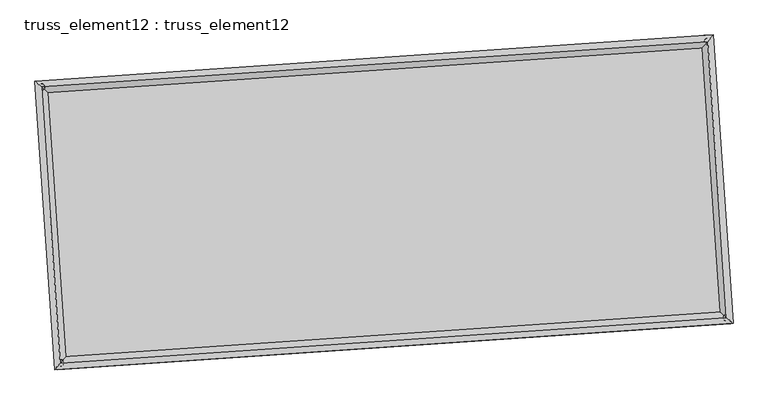
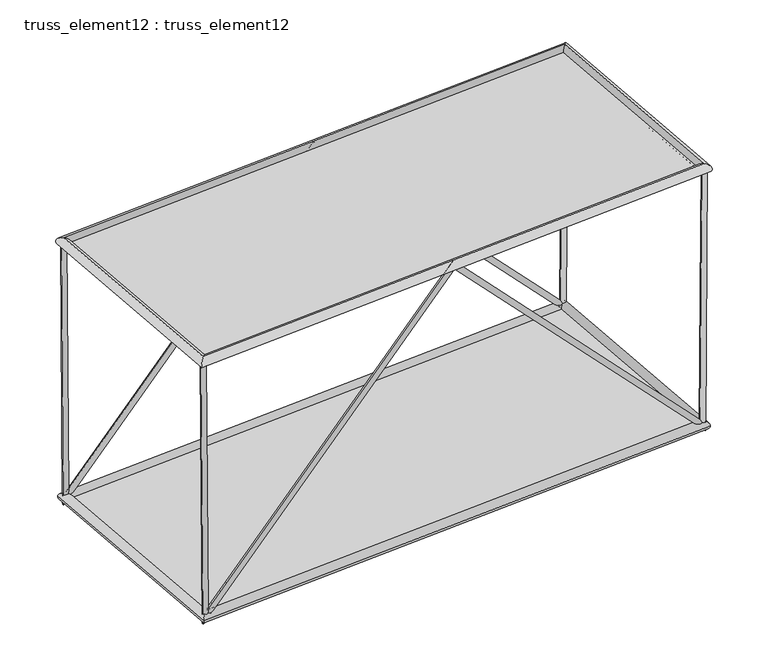
"""IFC4 building model written with IfcOpenShell, lengths in millimetres: plate geometry, truss_element12 : truss_element12."""

from ifc_helpers import new_model, si_unit, frame, origin, origin_with_axes, place, context, project, spatial, polyline, circle_curve, ellipse_curve, outline, extrude, source, transform, mapped, element, save
from ifc_brep_helpers import plane_surface, cylinder_surface, advanced_brep


def truss_element12_truss_element12_b90ce45a(model_context):
    return source(origin(), model_context, "Body", "SolidModel", [
        advanced_brep(
        [(-3700.9270944, 2273.7702742, 5000.2298034), (-3800.0278662, 2260.4091762, 4999.5100189), (-3665.8277368, 2276.163566, 123.2835915), (-3763.1591461, 2262.9231141, -123.2835915), (1063.4364737, 2598.6341149, 5071.9949176), (1063.8889024, 2592.0611712, 4927.7489342), (5793.2527985, 2921.1423104, 123.2875771), (5891.5081785, 2921.2381781, -123.2875771), (5827.8042267, 2923.4982409, 5000.2282154), (5927.8014861, 2923.7128808, 4999.5196659)],
        [
            (0, 1, circle_curve(frame((-3750.4774803, 2267.0897252, 4999.8699112), z_axis=(-0.007196807775674737, -0.0004907229645956758, 0.999973982235944), x_axis=(-0.13361103619871453, 0.9910337356173377, -0.0004752622967367017)), 50.0)),
            (1, 0, circle_curve(frame((-3750.4774803, 2267.0897252, 4999.8699112), z_axis=(-0.007196807775674737, -0.0004907229645956758, 0.999973982235944), x_axis=(-0.13361103619871453, 0.9910337356173377, -0.0004752622967367017)), 50.0)),
            (0, 2),
            (2, 3, ellipse_curve(frame((-3714.4934414, 2269.54334, 0.0), z_axis=(-0.9271277711546809, -0.06321731837243269, 0.36937469676678203), x_axis=(0.36851900189441095, 0.025127909867304916, 0.9292805461153525)), 132.9545126, 50.0)),
            (3, 1),
            (3, 2, ellipse_curve(frame((-3714.4934414, 2269.54334, 0.0), z_axis=(-0.9271277711546809, -0.06321731837243269, 0.36937469676678203), x_axis=(0.36851900189441095, 0.025127909867304916, 0.9292805461153525)), 132.9545126, 50.0)),
            (2, 4),
            (4, 5, ellipse_curve(frame((1063.6626881, 2595.347643, 4999.8719259), z_axis=(-0.9976833956449116, -0.06802823819938353, -2.9358585767190432e-05), x_axis=(2.9290573551987834e-05, 1.9972128666441766e-06, -0.9999999995690367)), 72.2800399, 50.0)),
            (5, 3),
            (5, 4, ellipse_curve(frame((1063.6626881, 2595.347643, 4999.8719259), z_axis=(-0.9976833956449116, -0.06802823819938353, -2.9358585767190432e-05), x_axis=(2.9290573551987834e-05, 1.9972128666441766e-06, -0.9999999995690367)), 72.2800399, 50.0)),
            (4, 6),
            (6, 7, ellipse_curve(frame((5842.3804885, 2921.1902443, 0.0), z_axis=(-0.9270962013206414, -0.06321516574545785, -0.3694542953013416), x_axis=(-0.36859841603069293, -0.02513332481537661, 0.9292489029766937)), 132.9633385, 50.0)),
            (7, 5),
            (7, 6, ellipse_curve(frame((5842.3804885, 2921.1902443, 0.0), z_axis=(-0.9270962013206414, -0.06321516574545785, -0.3694542953013416), x_axis=(-0.36859841603069293, -0.02513332481537661, 0.9292489029766937)), 132.9633385, 50.0)),
            (8, 9, circle_curve(frame((5877.8028564, 2923.6055609, 4999.8739406), z_axis=(0.007084473580336821, 0.0004830633228378769, 0.9999747881241386), x_axis=(-0.0021497673623656413, 0.9999975798082209, -0.00046784397887376233)), 50.0)),
            (9, 8, circle_curve(frame((5877.8028564, 2923.6055609, 4999.8739406), z_axis=(0.007084473580336821, 0.0004830633228378769, 0.9999747881241386), x_axis=(-0.0021497673623656413, 0.9999975798082209, -0.00046784397887376233)), 50.0)),
            (6, 8),
            (9, 7),
        ],
        [
            plane_surface(frame((-3750.4774803, 2317.0897192, 4999.894448), z_axis=(-0.007196807775676588, -0.0004907229645977611, 0.999973982235944), x_axis=(0.9999741026435836, -3.5317303099802163e-06, 0.0071968069091035095))),
            cylinder_surface(frame((-3750.4774803, 2267.0897252, 4999.8699112), z_axis=(-0.007196807775674737, -0.0004907229645956758, 0.999973982235944), x_axis=(-0.13361103619871453, 0.9910337356173377, -0.0004752622967367017)), 50.0),
            cylinder_surface(frame((-3714.4934414, 2269.54334, 0.0), z_axis=(-0.6901302351654753, -0.04705735730530593, -0.7221536288310727), x_axis=(-0.020411596190949132, 0.9987523751201103, -0.04557477298765516)), 50.0),
            cylinder_surface(frame((1063.6626881, 2595.347643, 4999.8719259), z_axis=(-0.6901725385637364, -0.04706024181322314, 0.7221130109982572), x_axis=(-0.11534659043872168, 0.9922791187440533, -0.04557756661655895)), 50.0),
            plane_surface(frame((5877.8028564, 2873.6055667, 4999.8980944), z_axis=(0.007084473580337363, 0.00048306332284136724, 0.9999747881241388), x_axis=(0.9999749048021604, -3.4223352329831814e-06, -0.007084472753714255))),
            cylinder_surface(frame((5842.3804885, 2921.1902443, 0.0), z_axis=(-0.007084473580336821, -0.0004830633228378769, -0.9999747881241386), x_axis=(-0.0021497673623656413, 0.9999975798082209, -0.00046784397887376233)), 50.0),
        ],
        [
            (0, [[1, 2]]),
            (1, [[-1, 3, 4, 5]]),
            (1, [[-2, -5, 6, -3]]),
            (2, [[-4, 7, 8, 9]]),
            (2, [[-6, -9, 10, -7]]),
            (3, [[-8, 11, 12, 13]]),
            (3, [[-10, -13, 14, -11]]),
            (4, [[15, 16]]),
            (5, [[-12, 17, -16, 18]]),
            (5, [[-14, -18, -15, -17]]),
        ],
    ),
        advanced_brep(
        [(-3428.8141415, -1716.9633101, 5000.2298034), (-3527.9149133, -1730.3244081, 4999.5100189), (-3393.7147839, -1714.5700183, 123.2835915), (-3491.0461931, -1727.8104702, -123.2835915), (1335.5494266, -1392.0994694, 5071.9949176), (1336.0018553, -1398.6724131, 4927.7489342), (6065.3657514, -1069.5912739, 123.2875771), (6163.6211314, -1069.4954062, -123.2875771), (6099.9171796, -1067.2353434, 5000.2282154), (6199.914439, -1067.0207035, 4999.5196659)],
        [
            (0, 1, circle_curve(frame((-3478.3645274, -1723.6438591, 4999.8699112), z_axis=(-0.007196807775674735, -0.0004907229645957192, 0.9999739822359441), x_axis=(-0.1336110361987148, 0.9910337356173377, -0.00047526229673666015)), 50.0)),
            (1, 0, circle_curve(frame((-3478.3645274, -1723.6438591, 4999.8699112), z_axis=(-0.007196807775674735, -0.0004907229645957192, 0.9999739822359441), x_axis=(-0.1336110361987148, 0.9910337356173377, -0.00047526229673666015)), 50.0)),
            (0, 2),
            (2, 3, ellipse_curve(frame((-3442.3804885, -1721.1902443, 0.0), z_axis=(-0.9271277711546809, -0.06321731837243283, 0.36937469676678225), x_axis=(0.36851900189441117, 0.025127909867304947, 0.9292805461153525)), 132.9545126, 50.0)),
            (3, 1),
            (3, 2, ellipse_curve(frame((-3442.3804885, -1721.1902443, 0.0), z_axis=(-0.9271277711546809, -0.06321731837243283, 0.36937469676678225), x_axis=(0.36851900189441117, 0.025127909867304947, 0.9292805461153525)), 132.9545126, 50.0)),
            (2, 4),
            (4, 5, ellipse_curve(frame((1335.775641, -1395.3859413, 4999.8719259), z_axis=(-0.9976833956449117, -0.06802823819938353, -2.9358585767110194e-05), x_axis=(2.9290573552141574e-05, 1.9972128665865233e-06, -0.9999999995690367)), 72.2800399, 50.0)),
            (5, 3),
            (5, 4, ellipse_curve(frame((1335.775641, -1395.3859413, 4999.8719259), z_axis=(-0.9976833956449117, -0.06802823819938353, -2.9358585767110194e-05), x_axis=(2.9290573552141574e-05, 1.9972128665865233e-06, -0.9999999995690367)), 72.2800399, 50.0)),
            (4, 6),
            (6, 7, ellipse_curve(frame((6114.4934414, -1069.54334, 0.0), z_axis=(-0.9270962013206415, -0.06321516574545775, -0.36945429530134144), x_axis=(-0.36859841603069265, -0.025133324815376546, 0.9292489029766939)), 132.9633385, 50.0)),
            (7, 5),
            (7, 6, ellipse_curve(frame((6114.4934414, -1069.54334, 0.0), z_axis=(-0.9270962013206415, -0.06321516574545775, -0.36945429530134144), x_axis=(-0.36859841603069265, -0.025133324815376546, 0.9292489029766939)), 132.9633385, 50.0)),
            (8, 9, circle_curve(frame((6149.9158093, -1067.1280234, 4999.8739406), z_axis=(0.0070844735803366, 0.0004830633228378691, 0.9999747881241385), x_axis=(-0.0021497673623655997, 0.999997579808221, -0.0004678439788737554)), 50.0)),
            (9, 8, circle_curve(frame((6149.9158093, -1067.1280234, 4999.8739406), z_axis=(0.0070844735803366, 0.0004830633228378691, 0.9999747881241385), x_axis=(-0.0021497673623655997, 0.999997579808221, -0.0004678439788737554)), 50.0)),
            (6, 8),
            (9, 7),
        ],
        [
            plane_surface(frame((-3478.3645274, -1673.6438651, 4999.894448), z_axis=(-0.007196807775676588, -0.0004907229645977664, 0.999973982235944), x_axis=(0.9999741026435836, -3.5317303099802163e-06, 0.0071968069091035095))),
            cylinder_surface(frame((-3478.3645274, -1723.6438591, 4999.8699112), z_axis=(-0.007196807775674733, -0.0004907229645957191, 0.9999739822359439), x_axis=(-0.1336110361987148, 0.9910337356173377, -0.00047526229673666015)), 50.0),
            cylinder_surface(frame((-3442.3804885, -1721.1902443, 0.0), z_axis=(-0.6901302351654753, -0.04705735730530598, -0.7221536288310728), x_axis=(-0.020411596190949188, 0.9987523751201103, -0.04557477298765517)), 50.0),
            cylinder_surface(frame((1335.775641, -1395.3859413, 4999.8719259), z_axis=(-0.6901725385637363, -0.04706024181322305, 0.7221130109982572), x_axis=(-0.11534659043872159, 0.9922791187440533, -0.04557756661655898)), 50.0),
            plane_surface(frame((6149.9158093, -1117.1280176, 4999.8980944), z_axis=(0.007084473580337363, 0.0004830633228413738, 0.9999747881241388), x_axis=(0.9999749048021604, -3.422335232539092e-06, -0.007084472753714255))),
            cylinder_surface(frame((6114.4934414, -1069.54334, 0.0), z_axis=(-0.007084473580336602, -0.0004830633228378692, -0.9999747881241388), x_axis=(-0.0021497673623655997, 0.999997579808221, -0.0004678439788737554)), 50.0),
        ],
        [
            (0, [[1, 2]]),
            (1, [[-1, 3, 4, 5]]),
            (1, [[-2, -5, 6, -3]]),
            (2, [[-4, 7, 8, 9]]),
            (2, [[-6, -9, 10, -7]]),
            (3, [[-8, 11, 12, 13]]),
            (3, [[-10, -13, 14, -11]]),
            (4, [[15, 16]]),
            (5, [[-12, 17, -16, 18]]),
            (5, [[-14, -18, -15, -17]]),
        ],
    ),
        advanced_brep(
        [(-3478.363464, -1723.6426805, 4909.8699112), (-3478.3655907, -1723.6450376, 5089.8699112), (-3750.4786938, 2267.0907485, 5089.8699112), (-3750.4762668, 2267.0887019, 4909.8699112), (5877.8038448, 2923.6067343, 5089.8739406), (5877.801868, 2923.6043874, 4909.8739406), (6149.9169478, -1067.1290519, 5089.8739406), (6149.9146708, -1067.126995, 4909.8739406)],
        [
            (0, 1, ellipse_curve(frame((-3478.3645274, -1723.6438591, 4999.8699112), z_axis=(-0.7535719234053955, 0.6573654662780861, -2.952390631555006e-07), x_axis=(-0.6573654662780204, -0.7535719234054526, -2.952390631554982e-07)), 127.2792206, 90.0)),
            (1, 2),
            (2, 3, ellipse_curve(frame((-3750.4774803, 2267.0897252, 4999.8699112), z_axis=(-0.6573654662780204, -0.7535719234054529, -2.9523906315549633e-07), x_axis=(0.7535719234053956, -0.6573654662780861, 2.952390631554988e-07)), 127.2792206, 90.0)),
            (3, 0),
            (1, 0, ellipse_curve(frame((-3478.3645274, -1723.6438591, 4999.8699112), z_axis=(-0.7535719234053955, 0.6573654662780861, -2.952390631555006e-07), x_axis=(-0.6573654662780204, -0.7535719234054526, -2.952390631554982e-07)), 127.2792206, 90.0)),
            (3, 2, ellipse_curve(frame((-3750.4774803, 2267.0897252, 4999.8699112), z_axis=(-0.6573654662780204, -0.7535719234054529, -2.9523906315549633e-07), x_axis=(0.7535719234053956, -0.6573654662780861, 2.952390631554988e-07)), 127.2792206, 90.0)),
            (2, 4),
            (4, 5, ellipse_curve(frame((5877.8028564, 2923.6055609, 4999.8739406), z_axis=(-0.7535719234053952, 0.6573654662780863, -2.9523906315549707e-07), x_axis=(-0.6573654662780207, -0.7535719234054524, -2.952390631554981e-07)), 127.2792206, 90.0)),
            (5, 3),
            (5, 4, ellipse_curve(frame((5877.8028564, 2923.6055609, 4999.8739406), z_axis=(-0.7535719234053952, 0.6573654662780863, -2.9523906315549707e-07), x_axis=(-0.6573654662780207, -0.7535719234054524, -2.952390631554981e-07)), 127.2792206, 90.0)),
            (4, 6),
            (6, 7, ellipse_curve(frame((6149.9158093, -1067.1280234, 4999.8739406), z_axis=(0.6573654662780206, 0.7535719234054526, 2.952390631554999e-07), x_axis=(-0.7535719234053955, 0.6573654662780862, -2.95239063155499e-07)), 127.2792206, 90.0)),
            (7, 5),
            (7, 6, ellipse_curve(frame((6149.9158093, -1067.1280234, 4999.8739406), z_axis=(0.6573654662780206, 0.7535719234054526, 2.952390631554999e-07), x_axis=(-0.7535719234053955, 0.6573654662780862, -2.95239063155499e-07)), 127.2792206, 90.0)),
            (6, 1),
            (0, 7),
        ],
        [
            cylinder_surface(frame((-3478.3645274, -1723.6438591, 4999.8699112), z_axis=(0.06802823822869845, -0.9976833960748769, 0.0), x_axis=(-0.9976833959946902, -0.06802823822323084, -1.267854125071923e-05)), 90.0),
            cylinder_surface(frame((-3750.4774803, 2267.0897252, 4999.8699112), z_axis=(-0.9976833960747897, -0.06802823822869523, -4.1753108725683143e-07), x_axis=(-0.06802823821848024, 0.9976833960002328, -1.2261010163493783e-05)), 90.0),
            cylinder_surface(frame((5877.8028564, 2923.6055609, 4999.8739406), z_axis=(-0.06802823822869786, 0.9976833960748768, 0.0), x_axis=(0.9976833960049053, 0.06802823822392676, -1.1843479076268334e-05)), 90.0),
            cylinder_surface(frame((6149.9158093, -1067.1280234, 4999.8739406), z_axis=(0.9976833960747897, 0.06802823822869523, 4.175310872568341e-07), x_axis=(0.06802823822869523, -0.9976833959995364, -1.2261010163493785e-05)), 90.0),
        ],
        [
            (0, [[1, 2, 3, 4]]),
            (0, [[5, -4, 6, -2]]),
            (1, [[-3, 7, 8, 9]]),
            (1, [[-6, -9, 10, -7]]),
            (2, [[-8, 11, 12, 13]]),
            (2, [[-10, -13, 14, -11]]),
            (3, [[-12, 15, -1, 16]]),
            (3, [[-14, -16, -5, -15]]),
        ],
    ),
        advanced_brep(
        [(-3358.7115243, -1625.2761972, 0.0), (-3526.0494527, -1817.1042913, 0.0), (-3810.4074885, 2353.2123043, 0.0), (-3618.5793943, 2185.8743758, 0.0), (5926.0494527, 3017.1042913, 0.0), (5758.7115243, 2825.2761972, 0.0), (6210.4074885, -1153.2123043, 0.0), (6018.5793943, -985.8743758, 0.0)],
        [
            (0, 1, ellipse_curve(frame((-3442.3804885, -1721.1902443, 0.0), z_axis=(-0.753571923405457, 0.6573654662780819, 0.0), x_axis=(-0.6573654662780819, -0.753571923405457, 0.0)), 127.2792206, 90.0)),
            (1, 2),
            (2, 3, ellipse_curve(frame((-3714.4934414, 2269.54334, 0.0), z_axis=(-0.6573654662780818, -0.7535719234054571, 0.0), x_axis=(0.7535719234054571, -0.6573654662780819, 0.0)), 127.2792206, 90.0)),
            (3, 0),
            (1, 0, ellipse_curve(frame((-3442.3804885, -1721.1902443, 0.0), z_axis=(-0.753571923405457, 0.6573654662780819, 0.0), x_axis=(-0.6573654662780819, -0.753571923405457, 0.0)), 127.2792206, 90.0)),
            (3, 2, ellipse_curve(frame((-3714.4934414, 2269.54334, 0.0), z_axis=(-0.6573654662780818, -0.7535719234054571, 0.0), x_axis=(0.7535719234054571, -0.6573654662780819, 0.0)), 127.2792206, 90.0)),
            (2, 4),
            (4, 5, ellipse_curve(frame((5842.3804885, 2921.1902443, 0.0), z_axis=(-0.753571923405457, 0.6573654662780819, 0.0), x_axis=(-0.657365466278082, -0.7535719234054571, 0.0)), 127.2792206, 90.0)),
            (5, 3),
            (5, 4, ellipse_curve(frame((5842.3804885, 2921.1902443, 0.0), z_axis=(-0.753571923405457, 0.6573654662780819, 0.0), x_axis=(-0.657365466278082, -0.7535719234054571, 0.0)), 127.2792206, 90.0)),
            (4, 6),
            (6, 7, ellipse_curve(frame((6114.4934414, -1069.54334, 0.0), z_axis=(0.6573654662780819, 0.753571923405457, 0.0), x_axis=(-0.7535719234054569, 0.6573654662780819, 0.0)), 127.2792206, 90.0)),
            (7, 5),
            (7, 6, ellipse_curve(frame((6114.4934414, -1069.54334, 0.0), z_axis=(0.6573654662780819, 0.753571923405457, 0.0), x_axis=(-0.7535719234054569, 0.6573654662780819, 0.0)), 127.2792206, 90.0)),
            (6, 1),
            (0, 7),
        ],
        [
            cylinder_surface(frame((-3442.3804885, -1721.1902443, 0.0), z_axis=(0.06802823822869875, -0.9976833960748768, 0.0), x_axis=(-0.9976833960748768, -0.06802823822869875, 0.0)), 90.0),
            cylinder_surface(frame((-3714.4934414, 2269.54334, 0.0), z_axis=(-0.9976833960748765, -0.06802823822870124, 0.0), x_axis=(-0.06802823822870124, 0.9976833960748765, 0.0)), 90.0),
            cylinder_surface(frame((5842.3804885, 2921.1902443, 0.0), z_axis=(-0.06802823822869838, 0.9976833960748768, 0.0), x_axis=(0.9976833960748768, 0.06802823822869838, 0.0)), 90.0),
            cylinder_surface(frame((6114.4934414, -1069.54334, 0.0), z_axis=(0.9976833960748767, 0.06802823822870088, 0.0), x_axis=(0.06802823822870088, -0.9976833960748767, 0.0)), 90.0),
        ],
        [
            (0, [[1, 2, 3, 4]]),
            (0, [[5, -4, 6, -2]]),
            (1, [[-3, 7, 8, 9]]),
            (1, [[-6, -9, 10, -7]]),
            (2, [[-8, 11, 12, 13]]),
            (2, [[-10, -13, 14, -11]]),
            (3, [[-12, 15, -1, 16]]),
            (3, [[-14, -16, -5, -15]]),
        ],
    ),
        extrude(outline(polyline([(-3442.3804885, -1721.1902443), (-3714.4934414, 2269.54334), (5842.3804885, 2921.1902443), (6114.4934414, -1069.54334), (-3442.3804885, -1721.1902443)])), origin_with_axes(), (0.0, 0.0, 1.0), 20.0),
        extrude(outline(polyline([(-2000.0, 4825.3185202), (2000.0, 4825.3185202), (2000.0, -4825.3185202), (-2000.0, -4825.3185202), (-2000.0, 4825.3185202)])), frame((1199.7191645, 599.9808509, 4999.8719259), z_axis=(-4.165638331012324e-07, -2.8403904271795323e-08, 0.9999999999999128), x_axis=(-0.06802823822869855, 0.9976833960748768, 0.0)), (0.0, 0.0, 1.0), 20.0),
    ])


if __name__ == "__main__":
    model = new_model("IFC4")
    model_context = context("Model", 3, world=origin())
    ifc_project = project(units=[si_unit("LENGTHUNIT", "METRE", prefix="MILLI")], contexts=[model_context])
    site = spatial("IfcSite", under=ifc_project)
    building = spatial("IfcBuilding", under=site)
    placement = place(None, origin())
    truss_element12_truss_element12_shape = truss_element12_truss_element12_b90ce45a(model_context)
    element("IfcPlate", 1, ObjectType="truss_element12 : truss_element12", at=placement, inside=building, context=model_context, shape_type="MappedRepresentation", body=[
        mapped(truss_element12_truss_element12_shape, transform((0.0, 0.0, 0.0), x_axis=(1.0, 0.0, 0.0), y_axis=(0.0, 1.0, 0.0), z_axis=(0.0, 0.0, 1.0))),
    ])
    save(model, "model.ifc")

# Revit data of these elements
# Type "truss_element12 : truss_element12"
#   steellbar1 = 90 mm
#   steelbar2 = 50 mm
#   offset1 = 5000 mm
#   M = Default Roof
# Element 1 (IfcPlate, "truss_element12 : truss_element12")
#   Materials on its faces: "Default Roof"
# Materials
#   "Default Roof": class "Miscellaneous", colour RGB 0 127 0, transparency 0, Comments = "Rendering appearance not upgraded Rendering appearance not upgraded ", Cost = 0
